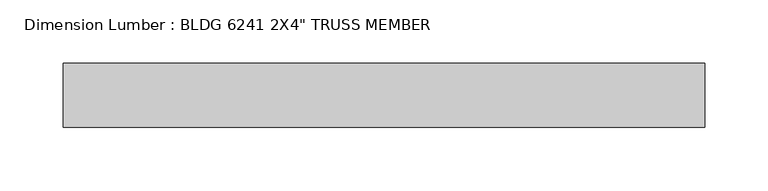
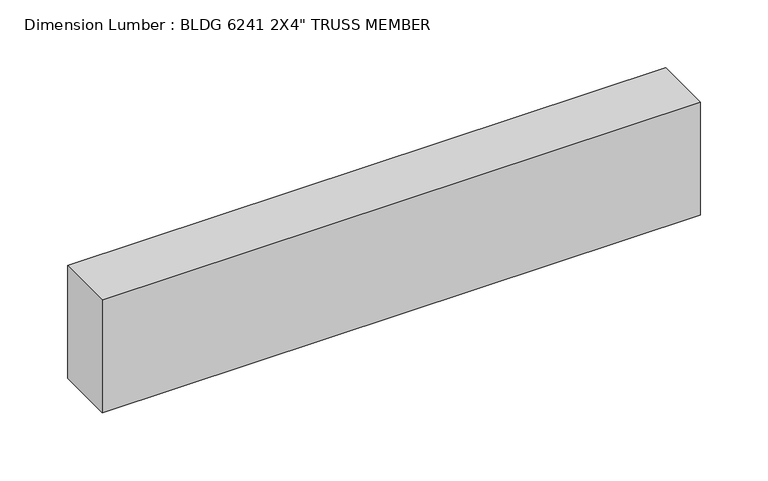
"""IFC4 building model written with IfcOpenShell, lengths in millimetres: beam geometry."""

from ifc_helpers import new_model, si_unit, frame, origin, place, context, project, spatial, polyline, outline, extrude, source, transform, mapped, element, save


def beam_ec111315(model_context):
    return source(origin(), model_context, "Body", "SweptSolid", [
        extrude(outline(polyline([(279.4, -25.4), (-228.6, -25.4), (-228.6, 25.4), (279.4, 25.4), (279.4, -25.4)])), frame((0.0, 0.0, -50.8), z_axis=(0.0, 0.0, 1.0), x_axis=(1.0, 0.0, 0.0)), (0.0, 0.0, 1.0), 101.6),
    ])


if __name__ == "__main__":
    model = new_model("IFC4")
    model_context = context("Model", 3, world=origin())
    ifc_project = project(units=[si_unit("LENGTHUNIT", "METRE", prefix="MILLI")], contexts=[model_context])
    site = spatial("IfcSite", under=ifc_project)
    building = spatial("IfcBuilding", under=site)
    placement = place(None, origin())
    beam_shape = beam_ec111315(model_context)
    element("IfcBeam", 1, ObjectType="Dimension Lumber : BLDG 6241 2X4\" TRUSS MEMBER", at=placement, inside=building, context=model_context, shape_type="MappedRepresentation", body=[
        mapped(beam_shape, transform((0.0, 0.0, 0.0), x_axis=(1.0, 0.0, 0.0), y_axis=(0.0, 1.0, 0.0), z_axis=(0.0, 0.0, 1.0))),
    ])
    save(model, "model.ifc")

# Revit data of these elements
# Type "Dimension Lumber : BLDG 6241 2X4\" TRUSS MEMBER"
#   Assembly Code = "B10"
#   A = 0.273472 SF
#   Length [instance default] = 5' - 0"
#   b = 0' - 2"
#   d = 0' - 4"
#   Structural Material [instance default] = Softwood, Lumber
# Element 1 (IfcBeam, "Dimension Lumber : BLDG 6241 2X4\" TRUSS MEMBER")
#   Materials on its faces: "Softwood, Lumber"
# Materials
#   "Softwood, Lumber": class "Wood", colour RGB 223 192 134, transparency 0, Description = "Pinus Echinata", Cost = 0
